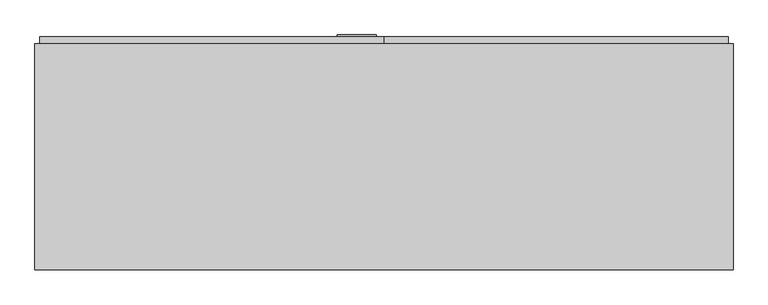
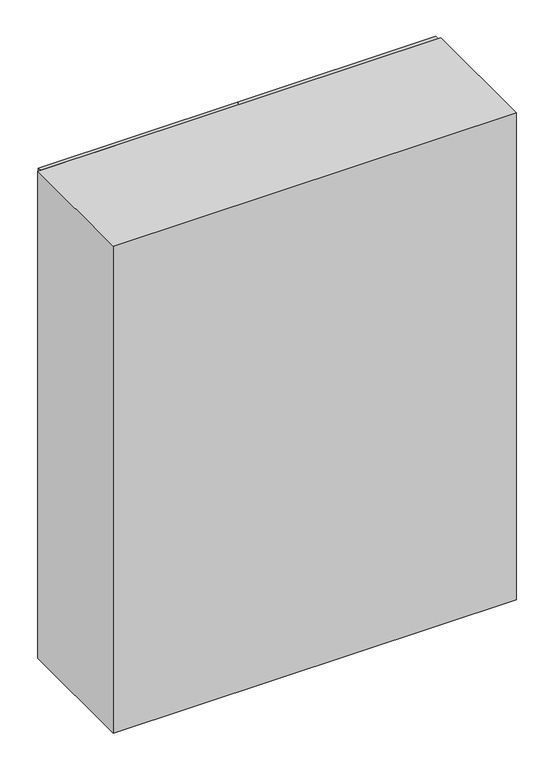
"""IFC4 building model written with IfcOpenShell, lengths in millimetres: furniture geometry, Armário - Closet - Porta com armação dupla 2 : Armário - Closet - Porta com armação dupla 2."""

from ifc_helpers import new_model, si_unit, frame, origin, origin_with_axes, place, context, project, spatial, polyline, outline, extrude, source, transform, mapped, element, save


def furniture_f3a75676(model_context):
    return source(origin(), model_context, "Body", "SweptSolid", [
        extrude(outline(polyline([(1205.0, -120.0), (1025.0, -120.0), (1025.0, -20.0), (1205.0, -20.0), (1205.0, -120.0)]), holes=[polyline([(1045.0, -100.0), (1185.0, -100.0), (1185.0, -60.0), (1045.0, -60.0), (1045.0, -100.0)])]), frame((0.0, 600.0, 0.0), z_axis=(0.0, 1.0, 0.0), x_axis=(0.0, 0.0, 1.0)), (0.0, 0.0, 1.0), 5.0),
        extrude(outline(polyline([(-60.0, 592.5), (-100.0, 592.5), (-100.0, 595.0), (-60.0, 595.0), (-60.0, 592.5)])), frame((0.0, 0.0, 1045.0), z_axis=(0.0, 0.0, 1.0), x_axis=(1.0, 0.0, 0.0)), (0.0, 0.0, 1.0), 140.0),
        extrude(outline(polyline([(900.0, 0.0), (-900.0, 0.0), (-900.0, 582.0), (900.0, 582.0), (900.0, 0.0)])), origin_with_axes(), (0.0, 0.0, 1.0), 2300.0),
        extrude(outline(polyline([(0.0, 582.0), (0.0, 600.0), (887.5, 600.0), (887.5, 582.0), (0.0, 582.0)])), frame((0.0, 0.0, 18.0), z_axis=(0.0, 0.0, 1.0), x_axis=(1.0, 0.0, 0.0)), (0.0, 0.0, 1.0), 2282.0),
        extrude(outline(polyline([(0.0, 582.0), (-887.5, 582.0), (-887.5, 600.0), (0.0, 600.0), (0.0, 582.0)])), frame((0.0, 0.0, 18.0), z_axis=(0.0, 0.0, 1.0), x_axis=(1.0, 0.0, 0.0)), (0.0, 0.0, 1.0), 2282.0),
    ])


if __name__ == "__main__":
    model = new_model("IFC4")
    model_context = context("Model", 3, world=origin())
    ifc_project = project(units=[si_unit("LENGTHUNIT", "METRE", prefix="MILLI")], contexts=[model_context])
    site = spatial("IfcSite", under=ifc_project)
    building = spatial("IfcBuilding", under=site)
    placement = place(None, origin())
    furniture_shape = furniture_f3a75676(model_context)
    element("IfcFurniture", 1, ObjectType="Armário - Closet - Porta com armação dupla 2 : Armário - Closet - Porta com armação dupla 2", at=placement, inside=building, context=model_context, shape_type="MappedRepresentation", body=[
        mapped(furniture_shape, transform((0.0, 0.0, 0.0), x_axis=(1.0, 0.0, 0.0), y_axis=(0.0, 1.0, 0.0), z_axis=(0.0, 0.0, 1.0))),
    ])
    save(model, "model.ifc")

# Revit data of these elements
# Type "Armário - Closet - Porta com armação dupla 2 : Armário - Closet - Porta com armação dupla 2"
#   Largura [instance default] = 1800 mm
#   Altura [instance default] = 2300 mm
#   Linear [instance default] = 600 mm
#   Material do closet = none
#   Material do puxador = none
